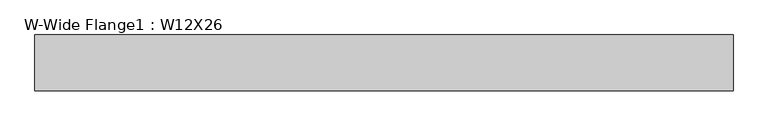
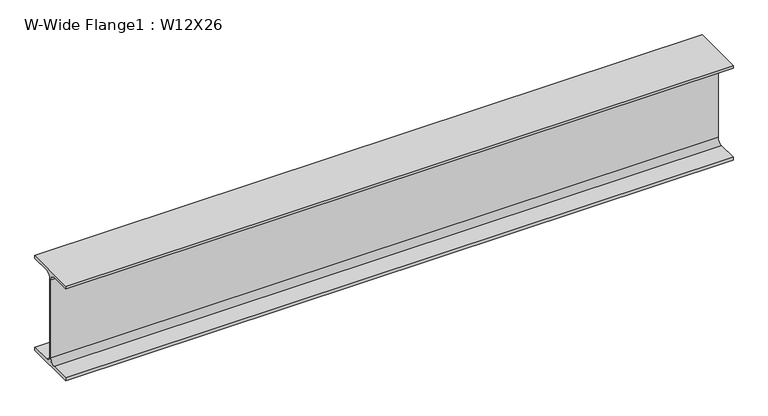
"""IFC4 building model written with IfcOpenShell, lengths in millimetres: beam geometry, W-Wide Flange1 : W12X26."""

from ifc_helpers import new_model, si_unit, point, frame, frame_2d, origin, place, context, project, spatial, polyline, circle_curve, trimmed, segment, composite_curve, outline, extrude, source, transform, mapped, element, save


def w_wide_flange1_w12x26_217799eb(model_context):
    return source(origin(), model_context, "Body", "SweptSolid", [
        extrude(outline(composite_curve([segment(polyline([(82.423, -145.288), (82.423, -154.94), (-82.423, -154.94), (-82.423, -145.288), (-20.2565, -145.288)]), True, "CONTINUOUS"), segment(trimmed(circle_curve(frame_2d((-20.2565, -127.9525)), 17.3355), [point((-20.2565, -145.288))], [point((-2.921, -127.9525))], True, "CARTESIAN"), True, "CONTINUOUS"), segment(polyline([(-2.921, -127.9525), (-2.921, 127.9525)]), True, "CONTINUOUS"), segment(trimmed(circle_curve(frame_2d((-20.2565, 127.9525)), 17.3355), [point((-2.921, 127.9525))], [point((-20.2565, 145.288))], True, "CARTESIAN"), True, "CONTINUOUS"), segment(polyline([(-20.2565, 145.288), (-82.423, 145.288), (-82.423, 154.94), (82.423, 154.94), (82.423, 145.288), (20.2565, 145.288)]), True, "CONTINUOUS"), segment(trimmed(circle_curve(frame_2d((20.2565, 127.9525)), 17.3355), [point((20.2565, 145.288))], [point((2.921, 127.9525))], True, "CARTESIAN"), True, "CONTINUOUS"), segment(polyline([(2.921, 127.9525), (2.921, -127.9525)]), True, "CONTINUOUS"), segment(trimmed(circle_curve(frame_2d((20.2565, -127.9525)), 17.3355), [point((2.921, -127.9525))], [point((20.2565, -145.288))], True, "CARTESIAN"), True, "CONTINUOUS"), segment(polyline([(20.2565, -145.288), (82.423, -145.288)]), True, "CONTINUOUS")], self_intersect=False)), frame((-1021.8198801, 0.0, 0.0), z_axis=(1.0, 0.0, 0.0), x_axis=(0.0, 1.0, 0.0)), (0.0, 0.0, 1.0), 2061.1607427),
    ])


if __name__ == "__main__":
    model = new_model("IFC4")
    model_context = context("Model", 3, world=origin())
    ifc_project = project(units=[si_unit("LENGTHUNIT", "METRE", prefix="MILLI")], contexts=[model_context])
    site = spatial("IfcSite", under=ifc_project)
    building = spatial("IfcBuilding", under=site)
    placement = place(None, origin())
    w_wide_flange1_w12x26_shape = w_wide_flange1_w12x26_217799eb(model_context)
    element("IfcBeam", 1, ObjectType="W-Wide Flange1 : W12X26", at=placement, inside=building, context=model_context, shape_type="MappedRepresentation", body=[
        mapped(w_wide_flange1_w12x26_shape, transform((0.0, 0.0, 0.0), x_axis=(1.0, 0.0, 0.0), y_axis=(0.0, 1.0, 0.0), z_axis=(0.0, 0.0, 1.0))),
    ])
    save(model, "model.ifc")

# Revit data of these elements
# Type "W-Wide Flange1 : W12X26"
#   Assembly Code = "B10"
#   W = 26
#   Start Extension Calculation [instance default] = 10' - 0"
#   Start Extension [instance default] = -0' - 0 1/2"
#   End Extension Calculation [instance default] = 10' - 0"
#   End Extension [instance default] = -0' - 0 1/2"
#   Length [instance default] = 5' - 0"
#   bf = 0' - 6.49"
#   d = 1' - 0.2"
#   k = 0' - 1 1/16"
#   k2 = 0' - 0.6825"
#   tf = 0' - 0.38"
#   tw = 0' - 0.23"
#   A = 0.053125 SF
#   Structural Material [instance default] = Metal - Steel - ASTM A992
# Element 1 (IfcBeam, "W-Wide Flange1 : W12X26")
#   Materials on its faces: "Metal - Steel - ASTM A992"
# Materials
#   "Metal - Steel - ASTM A992": class "Metal", colour RGB 199 199 199, transparency 0
